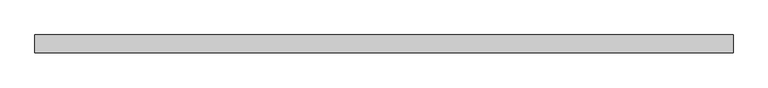
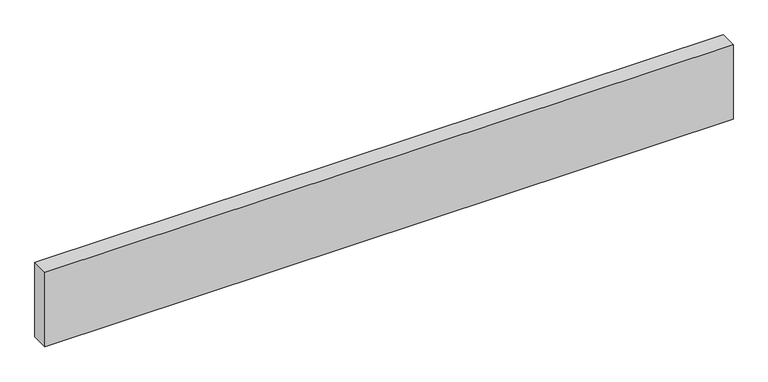
"""IFC4 building model written with IfcOpenShell, lengths in millimetres: proxy geometry, Blocking012 3310 : Blocking012 3310."""

from ifc_helpers import new_model, si_unit, frame, origin, place, context, project, spatial, polyline, outline, extrude, source, transform, mapped, element, save


def generic_models_9b28f469(model_context):
    return source(origin(), model_context, "Body", "SweptSolid", [
        extrude(outline(polyline([(3694.2883192, 9699.862737), (3694.2883192, 9750.662737), (5694.2883192, 9750.662737), (5694.2883192, 9699.862737), (3694.2883192, 9699.862737)])), frame((0.0, 0.0, 39528.496), z_axis=(0.0, 0.0, 1.0), x_axis=(1.0, 0.0, 0.0)), (0.0, 0.0, 1.0), 228.6),
    ])


if __name__ == "__main__":
    model = new_model("IFC4")
    model_context = context("Model", 3, world=origin())
    ifc_project = project(units=[si_unit("LENGTHUNIT", "METRE", prefix="MILLI")], contexts=[model_context])
    site = spatial("IfcSite", under=ifc_project)
    building = spatial("IfcBuilding", under=site)
    placement = place(None, origin())
    generic_models_shape = generic_models_9b28f469(model_context)
    element("IfcBuildingElementProxy", 1, Name="Blocking012 3310 : Blocking012 3310", ObjectType="Blocking012 3310 : Blocking012 3310", at=placement, inside=building, context=model_context, shape_type="MappedRepresentation", body=[
        mapped(generic_models_shape, transform((0.0, 0.0, 0.0), x_axis=(1.0, 0.0, 0.0), y_axis=(0.0, 1.0, 0.0), z_axis=(0.0, 0.0, 1.0))),
    ])
    save(model, "model.ifc")

# Revit data of these elements
# Type "Blocking012 3310 : Blocking012 3310"
#   NameOverride = "Blocking012"
# Element 1 (IfcBuildingElementProxy, "Blocking012 3310 : Blocking012 3310")
#   Materials on its faces: "WOOD BLOCKING AS REQUIRED"
# Materials
#   "WOOD BLOCKING AS REQUIRED": class "Unassigned", colour RGB 166 124 85, transparency 0, Cost = 0
